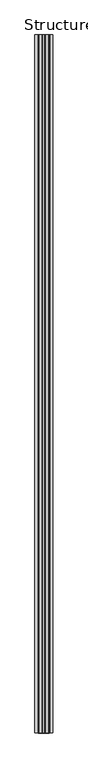
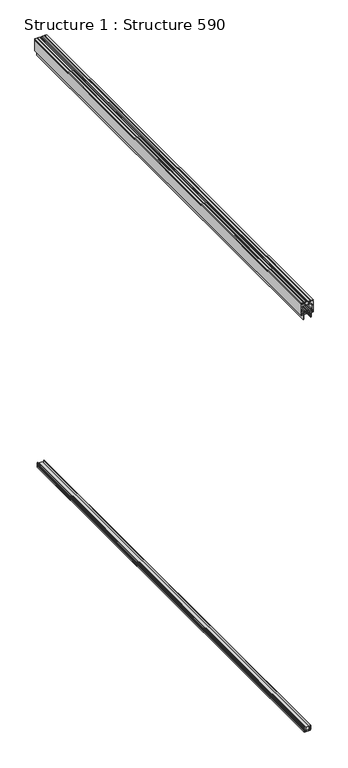
"""IFC4 building model written with IfcOpenShell, lengths in millimetres: proxy geometry, Structure 1 : Structure 590."""

from ifc_helpers import new_model, si_unit, frame, origin, place, context, project, spatial, polyline, outline, extrude, source, transform, mapped, element, save


def structure_1_structure_590_6f9aee44(model_context):
    return source(origin(), model_context, "Body", "SweptSolid", [
        extrude(outline(polyline([(37604.2015618, 7571.6095342), (37604.2015618, 7597.6133363), (37606.7094313, 7600.1212059), (37611.5111794, 7600.1212059), (37613.3758754, 7599.646635), (37616.0506024, 7600.4492528), (37616.0506024, 7599.646635), (37618.7253294, 7600.4492528), (37618.7253294, 7599.646635), (37621.4000564, 7600.4492528), (37621.4000564, 7599.646635), (37624.0747835, 7600.4492528), (37624.0747835, 7599.646635), (37626.7495105, 7599.646635), (37628.5339519, 7597.8621935), (37606.8963912, 7597.8621935), (37606.8963912, 7591.5121935), (37609.4991896, 7591.5121935), (37609.4991896, 7577.710677), (37606.8963912, 7577.710677), (37606.8963912, 7571.360677), (37628.5339519, 7571.360677), (37626.7495105, 7569.5762356), (37624.0747835, 7569.5762356), (37624.0747835, 7568.7736177), (37621.4000564, 7569.5762356), (37621.4000564, 7568.7736177), (37618.7253294, 7569.5762356), (37618.7253294, 7568.7736177), (37616.0506024, 7569.5762356), (37616.0506024, 7568.7736177), (37613.3758754, 7569.5762356), (37611.5111794, 7569.1016647), (37606.7094313, 7569.1016647), (37604.2015618, 7571.6095342)])), frame((0.0, -3747.9491938, 0.0), z_axis=(0.0, 1.0, 0.0), x_axis=(0.0, 0.0, 1.0)), (0.0, 0.0, 1.0), 2000.0),
        extrude(outline(polyline([(7591.5121935, -3747.9491938), (7577.710677, -3747.9491938), (7577.710677, -1747.9491938), (7591.5121935, -1747.9491938), (7591.5121935, -3747.9491938)])), frame((0.0, 0.0, 37609.4991896), z_axis=(0.0, 0.0, 1.0), x_axis=(1.0, 0.0, 0.0)), (0.0, 0.0, 1.0), 14.5755939),
        extrude(outline(polyline([(39531.1229547, 7576.278047), (39529.4644176, 7574.6195098), (39526.8565583, 7574.6195098), (39524.5631085, 7573.2953859), (39523.4368951, 7573.9983641), (39522.1597941, 7573.9983641), (39521.1460972, 7572.3826414), (39522.1017999, 7570.6701494), (39523.3870211, 7570.6701494), (39524.5633406, 7571.4489628), (39526.8567011, 7570.1248905), (39526.8567011, 7569.0544861), (39533.4499672, 7569.0544861), (39533.4499672, 7571.5345488), (39535.108298, 7571.5345488), (39535.108298, 7566.5396168), (39496.0572836, 7566.5396168), (39496.0572836, 7569.5360568), (39498.7320107, 7569.5360568), (39498.7320107, 7568.7334389), (39501.4067377, 7569.5360568), (39501.4067377, 7568.7334389), (39504.0814647, 7569.5360568), (39504.0814647, 7568.7334389), (39506.7561917, 7569.5360568), (39506.7561917, 7568.7334389), (39509.4309187, 7569.5360568), (39511.5829573, 7569.0544861), (39518.6052323, 7569.0544861), (39518.6052323, 7581.3077856), (39522.4568392, 7581.3077856), (39522.4568392, 7579.9700892), (39521.1194757, 7579.9700892), (39521.1194757, 7576.278047), (39529.464624, 7576.278047), (39529.464624, 7579.9700892), (39528.1272605, 7579.9700892), (39528.1272605, 7581.2798644), (39531.1229547, 7581.2798644), (39531.1229547, 7576.278047)])), frame((0.0, -3747.9491938, 0.0), z_axis=(0.0, 1.0, 0.0), x_axis=(0.0, 0.0, 1.0)), (0.0, 0.0, 1.0), 2000.0),
        extrude(outline(polyline([(39528.1272605, 7587.9430061), (39528.1272605, 7589.2527814), (39529.464624, 7589.2527814), (39529.464624, 7592.9448236), (39521.1194757, 7592.9448236), (39521.1194757, 7589.2527814), (39522.4568392, 7589.2527814), (39522.4568392, 7587.9150849), (39518.6052323, 7587.9150849), (39518.6052323, 7600.1683845), (39511.5829573, 7600.1683845), (39509.4309187, 7599.6868137), (39506.7561917, 7600.4894316), (39506.7561917, 7599.6868137), (39504.0814647, 7600.4894316), (39504.0814647, 7599.6868137), (39501.4067377, 7600.4894316), (39501.4067377, 7599.6868137), (39498.7320107, 7600.4894316), (39498.7320107, 7599.6868137), (39496.0572836, 7599.6868137), (39496.0572836, 7602.6832538), (39535.108298, 7602.6832538), (39535.108298, 7597.6883218), (39533.4499672, 7597.6883218), (39533.4499672, 7600.1683845), (39526.8567011, 7600.1683845), (39526.8567011, 7599.0979801), (39524.5633406, 7597.7739078), (39523.3870211, 7598.5527211), (39522.1017999, 7598.5527211), (39521.1460972, 7596.8402291), (39522.1597941, 7595.2245065), (39523.4368951, 7595.2245065), (39524.5631085, 7595.9274847), (39526.8565583, 7594.6033608), (39529.4644176, 7594.6033608), (39531.1229547, 7592.9448236), (39531.1229547, 7587.9430061), (39528.1272605, 7587.9430061)])), frame((0.0, -3747.9491938, 0.0), z_axis=(0.0, 1.0, 0.0), x_axis=(0.0, 0.0, 1.0)), (0.0, 0.0, 1.0), 2000.0),
        extrude(outline(polyline([(39569.2191527, 7610.0127866), (39572.946, 7610.0127866), (39572.946, 7602.553602), (39570.3642897, 7602.553602), (39571.2713147, 7601.0889604), (39570.4312008, 7599.9217089), (39569.4371392, 7600.4591368), (39567.3628315, 7600.8754823), (39565.7479015, 7599.2963484), (39566.1791001, 7597.1105383), (39568.0762045, 7596.1990469), (39569.7056116, 7597.1976803), (39572.946, 7597.1976803), (39572.946, 7590.3137987), (39568.7468805, 7590.3137987), (39570.179738, 7593.0028017), (39560.2371417, 7593.0028017), (39561.4571698, 7590.0583322), (39560.7401259, 7589.4520424), (39557.7331491, 7589.2177522), (39558.5286351, 7591.344992), (39559.6684085, 7591.344992), (39559.6684085, 7592.9190996), (39558.642991, 7592.9190996), (39558.642991, 7605.0636194), (39556.6369457, 7607.0696647), (39554.484732, 7607.0696647), (39552.7250638, 7606.0537198), (39551.5214367, 7606.0537198), (39551.5214367, 7607.0698544), (39548.8467096, 7607.0698544), (39548.8467096, 7606.0539094), (39547.643192, 7606.0539094), (39545.8835238, 7607.0698544), (39528.7060153, 7607.0698544), (39528.7060153, 7605.5983883), (39525.309112, 7605.5983883), (39525.309112, 7606.6685454), (39527.0476845, 7606.6685454), (39527.0476845, 7608.0062419), (39518.7560308, 7608.0062419), (39518.7560308, 7606.6685454), (39520.4946033, 7606.6685454), (39520.4946033, 7605.5985215), (39518.167724, 7605.5985215), (39517.0977, 7606.6685454), (39517.0977, 7610.0127866), (39565.911468, 7610.0127866), (39565.911468, 7606.4010061), (39570.9399547, 7606.4010061), (39569.2191527, 7610.0127866)])), frame((0.0, -3747.9491938, 0.0), z_axis=(0.0, 1.0, 0.0), x_axis=(0.0, 0.0, 1.0)), (0.0, 0.0, 1.0), 2000.0),
        extrude(outline(polyline([(39568.3263457, 7579.2446421), (39569.6322371, 7576.3378733), (39560.756306, 7576.3378733), (39561.8121843, 7578.6426561), (39561.8121843, 7579.5050905), (39558.6894612, 7581.9104975), (39558.6894612, 7587.4681948), (39561.7720192, 7589.8561724), (39561.7720192, 7591.0782964), (39560.819854, 7592.8149622), (39569.5290902, 7592.8149622), (39568.3928513, 7590.0578173), (39571.7499547, 7587.354265), (39571.7499547, 7581.9331644), (39568.3263457, 7579.2446421)])), frame((0.0, -3747.9491938, 0.0), z_axis=(0.0, 1.0, 0.0), x_axis=(0.0, 0.0, 1.0)), (0.0, 0.0, 1.0), 2000.0),
        extrude(outline(polyline([(39565.911468, 7562.8218644), (39565.911468, 7559.210084), (39517.0977, 7559.210084), (39517.0977, 7562.5543251), (39518.167724, 7563.6243491), (39520.4946033, 7563.6243491), (39520.4946033, 7562.5543251), (39518.7560308, 7562.5543251), (39518.7560308, 7561.2166287), (39527.0476845, 7561.2166287), (39527.0476845, 7562.5543251), (39525.309112, 7562.5543251), (39525.309112, 7563.6244823), (39528.7060153, 7563.6244823), (39528.7060153, 7562.1530162), (39545.8835238, 7562.1530162), (39547.643192, 7563.1689611), (39548.8467096, 7563.1689611), (39548.8467096, 7562.1530162), (39551.5214367, 7562.1530162), (39551.5214367, 7563.1691508), (39552.7250638, 7563.1691508), (39554.484732, 7562.1532059), (39556.6369457, 7562.1532059), (39558.642991, 7564.1592511), (39558.642991, 7576.303771), (39559.6684085, 7576.303771), (39559.6684085, 7577.8778786), (39558.5286351, 7577.8778786), (39557.7331491, 7580.0051183), (39560.7401259, 7579.7708282), (39561.4571698, 7579.1645383), (39560.2371417, 7576.2200689), (39570.179738, 7576.2200689), (39568.7468805, 7578.9090719), (39572.946, 7578.9090719), (39572.946, 7572.0251903), (39569.7056116, 7572.0251903), (39568.0762045, 7573.0238237), (39566.1791001, 7572.1123323), (39565.7479015, 7569.9265222), (39567.3628315, 7568.3473882), (39569.4371392, 7568.7637338), (39570.4312008, 7569.3011617), (39571.2713147, 7568.1339101), (39570.3642897, 7566.6692685), (39572.946, 7566.6692685), (39572.946, 7559.210084), (39569.2191527, 7559.210084), (39570.9399547, 7562.8218644), (39565.911468, 7562.8218644)])), frame((0.0, -3747.9491938, 0.0), z_axis=(0.0, 1.0, 0.0), x_axis=(0.0, 0.0, 1.0)), (0.0, 0.0, 1.0), 2000.0),
    ])


if __name__ == "__main__":
    model = new_model("IFC4")
    model_context = context("Model", 3, world=origin())
    ifc_project = project(units=[si_unit("LENGTHUNIT", "METRE", prefix="MILLI")], contexts=[model_context])
    site = spatial("IfcSite", under=ifc_project)
    building = spatial("IfcBuilding", under=site)
    placement = place(None, origin())
    structure_1_structure_590_shape = structure_1_structure_590_6f9aee44(model_context)
    element("IfcBuildingElementProxy", 1, Name="Structure 1 : Structure 590", ObjectType="Structure 1 : Structure 590", at=placement, inside=building, context=model_context, shape_type="MappedRepresentation", body=[
        mapped(structure_1_structure_590_shape, transform((0.0, 0.0, 0.0), x_axis=(1.0, 0.0, 0.0), y_axis=(0.0, 1.0, 0.0), z_axis=(0.0, 0.0, 1.0))),
    ])
    save(model, "model.ifc")

# Revit data of these elements
# Type "Structure 1 : Structure 590"
#   NameOverride = "Structure"
# Element 1 (IfcBuildingElementProxy, "Structure 1 : Structure 590")
#   Materials on its faces: "FLEETWOOD SLIDING DOOR SERIES 3070 (SEE ELEVATIONS FOR OPERABILITY)", "RUBBER", "IfcSurfaceStyle #584"
# Materials
#   "FLEETWOOD SLIDING DOOR SERIES 3070 (SEE ELEVATIONS FOR OPERABILITY)": class "Unassigned", colour RGB 143 136 136, transparency 0, Cost = 0
#   "RUBBER": class "Unassigned", colour RGB 70 70 70, transparency 0, Cost = 0
#   "IfcSurfaceStyle #584": class "Unassigned", colour RGB 169 181 186, transparency 0
